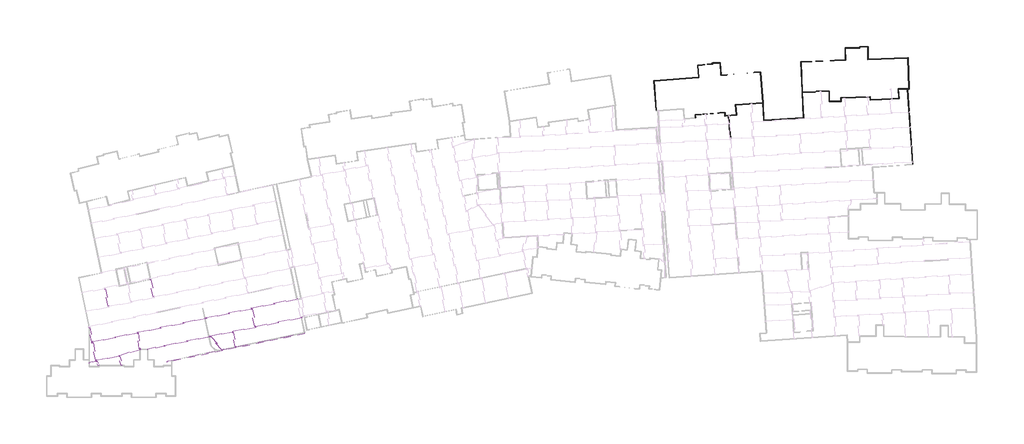
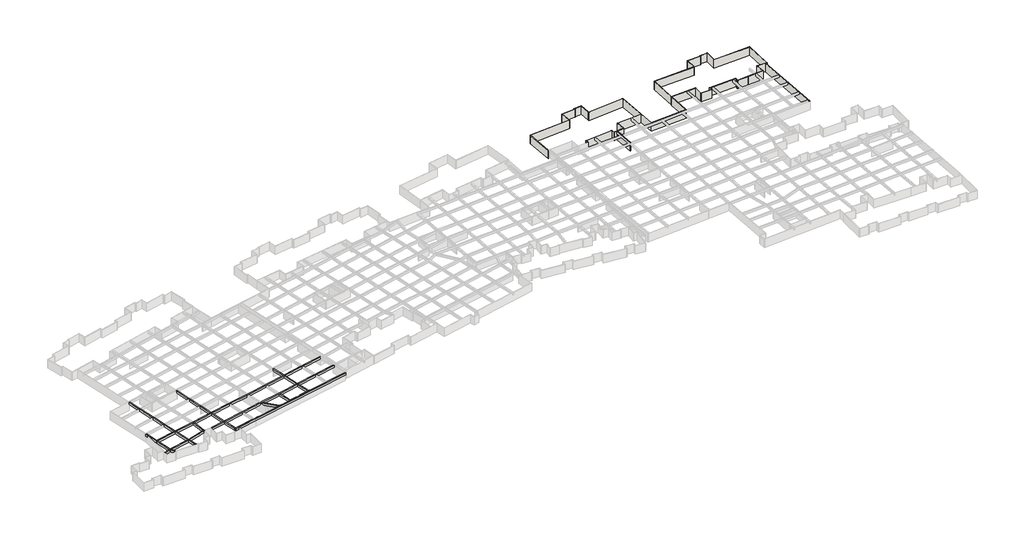
# One storey, part 7 of 14: 39 walls, 16 beams.
"""IFC4 building model written with IfcOpenShell, lengths in millimetres."""

from ifc_helpers import new_model, si_unit, frame, origin, origin_with_axes, place, context, project, spatial, polyline, outline, extrude, faceted_brep, element, save

model = new_model("IFC4")

# Units and contexts
model_context = context("Model", 3, world=origin())
ifc_project = project(units=[si_unit("LENGTHUNIT", "METRE", prefix="MILLI")], contexts=[model_context])

# Site, building, storey
site = spatial("IfcSite", under=ifc_project)
building = spatial("IfcBuilding", under=site)
storey = spatial("IfcBuildingStorey", under=building, Name="户型图", Elevation=0.0)

# Beams
placement = place(None, origin())
element("IfcBeam", 1, ObjectType="混凝土 - 矩形梁 : KL_beam", at=placement, inside=storey, context=model_context, shape_type="Brep", body=[
    faceted_brep([(-263201.3012877, -185738.5958614, 3300.0), (-263118.1366114, -186129.8549017, 3300.0), (-263118.1366114, -186129.8549017, 2500.0), (-263201.3012877, -185738.5958614, 2500.0), (-270867.2111578, -187368.0353054, 3300.0), (-271258.4701981, -187451.1999817, 3300.0), (-278694.4077882, -189031.7573087, 3300.0), (-279085.6668285, -189114.921985, 3300.0), (-286512.5798142, -190693.5610731, 3300.0), (-286903.8388545, -190776.7257494, 3300.0), (-294373.2864186, -192364.4058412, 3300.0), (-294764.5454589, -192447.5705175, 3300.0), (-302149.0676913, -194017.1991728, 3300.0), (-302540.3269101, -194100.3638871, 3300.0), (-310014.318982, -195689.0099438, 3300.0), (-310405.5780223, -195772.1746202, 3300.0), (-317795.331615, -197342.9152354, 3300.0), (-318186.5906553, -197426.0799118, 3300.0), (-325566.4629617, -198994.7201948, 3300.0), (-325957.722002, -199077.8848711, 3300.0), (-333450.1072491, -200670.4405179, 3300.0), (-333841.3662894, -200753.6051942, 3300.0), (-333758.2016131, -201144.8642345, 3300.0), (-333366.9425728, -201061.6995582, 3300.0), (-325874.5573256, -199469.1439114, 3300.0), (-325483.2982853, -199385.979235, 3300.0), (-318121.2886173, -197821.135773, 3300.0), (-317728.535031, -197737.6534211, 3300.0), (-310322.4133459, -196163.4336605, 3300.0), (-309931.1543056, -196080.2689841, 3300.0), (-302456.7885265, -194491.5434934, 3300.0), (-302065.5293077, -194408.3787792, 3300.0), (-294681.3807826, -192838.8295578, 3300.0), (-294290.1217423, -192755.6648815, 3300.0), (-286820.6741782, -191167.9847897, 3300.0), (-286429.4151379, -191084.8201134, 3300.0), (-279002.5021521, -189506.1810253, 3300.0), (-278611.2431118, -189423.016349, 3300.0), (-271175.3055217, -187842.459022, 3300.0), (-270784.0464815, -187759.2943457, 3300.0), (-333758.2016131, -201144.8642345, 2500.0), (-333366.9425728, -201061.6995582, 2500.0), (-325874.5573256, -199469.1439114, 2500.0), (-325483.2982853, -199385.979235, 2500.0), (-318121.2886173, -197821.135773, 2500.0), (-317728.535031, -197737.6534211, 2500.0), (-310322.4133459, -196163.4336605, 2500.0), (-309931.1543056, -196080.2689841, 2500.0), (-302456.7885265, -194491.5434934, 2500.0), (-302065.5293077, -194408.3787792, 2500.0), (-294681.3807826, -192838.8295578, 2500.0), (-294290.1217423, -192755.6648815, 2500.0), (-286820.6741782, -191167.9847897, 2500.0), (-286429.4151379, -191084.8201134, 2500.0), (-279002.5021521, -189506.1810253, 2500.0), (-278611.2431118, -189423.016349, 2500.0), (-271175.3055217, -187842.459022, 2500.0), (-270784.0464815, -187759.2943457, 2500.0), (-333841.3662894, -200753.6051942, 2500.0), (-333450.1072491, -200670.4405179, 2500.0), (-325957.722002, -199077.8848711, 2500.0), (-325566.4629617, -198994.7201948, 2500.0), (-318186.5906553, -197426.0799118, 2500.0), (-317795.331615, -197342.9152354, 2500.0), (-310405.5780223, -195772.1746202, 2500.0), (-310014.318982, -195689.0099438, 2500.0), (-302540.3269101, -194100.3638871, 2500.0), (-302149.0676913, -194017.1991728, 2500.0), (-294764.5454589, -192447.5705175, 2500.0), (-294373.2864186, -192364.4058412, 2500.0), (-286903.8388545, -190776.7257494, 2500.0), (-286512.5798142, -190693.5610731, 2500.0), (-279085.6668285, -189114.921985, 2500.0), (-278694.4077882, -189031.7573087, 2500.0), (-271258.4701981, -187451.1999817, 2500.0), (-270867.2111578, -187368.0353054, 2500.0)], [[[0, 1, 2, 3]], [[1, 0, 4, 5, 6, 7, 8, 9, 10, 11, 12, 13, 14, 15, 16, 17, 18, 19, 20, 21, 22, 23, 24, 25, 26, 27, 28, 29, 30, 31, 32, 33, 34, 35, 36, 37, 38, 39]], [[2, 1, 39, 38, 37, 36, 35, 34, 33, 32, 31, 30, 29, 28, 27, 26, 25, 24, 23, 22, 40, 41, 42, 43, 44, 45, 46, 47, 48, 49, 50, 51, 52, 53, 54, 55, 56, 57]], [[3, 2, 57, 56, 55, 54, 53, 52, 51, 50, 49, 48, 47, 46, 45, 44, 43, 42, 41, 40, 58, 59, 60, 61, 62, 63, 64, 65, 66, 67, 68, 69, 70, 71, 72, 73, 74, 75]], [[0, 3, 75, 74, 73, 72, 71, 70, 69, 68, 67, 66, 65, 64, 63, 62, 61, 60, 59, 58, 21, 20, 19, 18, 17, 16, 15, 14, 13, 12, 11, 10, 9, 8, 7, 6, 5, 4]], [[22, 21, 58, 40]]]),
])
element("IfcBeam", 2, ObjectType="混凝土 - 矩形梁 : KL_beam", at=placement, inside=storey, context=model_context, shape_type="Brep", body=[
    faceted_brep([(-324374.5463738, -205804.6094179, 3300.0), (-324476.8521438, -205417.4189427, 3300.0), (-324604.4476356, -205444.5402017, 3300.0), (-332096.8328827, -207037.0958485, 3300.0), (-332488.091923, -207120.2605249, 3300.0), (-332483.9504903, -207139.7444339, 3300.0), (-332404.9272467, -207511.5195652, 3300.0), (-332199.0452178, -207467.757989, 3300.0), (-331946.3573579, -207414.0475263, 3300.0), (-324510.9984157, -205833.6131948, 3300.0), (-324374.5463738, -205804.6094179, 2500.0), (-332404.9272467, -207511.5195652, 2500.0), (-332199.0452178, -207467.757989, 2500.0), (-331946.3573579, -207414.0475263, 2500.0), (-324510.9984157, -205833.6131948, 2500.0), (-324476.8521438, -205417.4189427, 2500.0), (-332483.9504903, -207139.7444339, 2500.0), (-332488.091923, -207120.2605249, 2500.0), (-332096.8328827, -207037.0958485, 2500.0), (-324604.4476356, -205444.5402017, 2500.0)], [[[0, 1, 2, 3, 4, 5, 6, 7, 8, 9]], [[10, 0, 9, 8, 7, 6, 11, 12, 13, 14]], [[15, 10, 14, 13, 12, 11, 16, 17, 18, 19]], [[1, 15, 19, 18, 17, 4, 3, 2]], [[1, 0, 10, 15]], [[6, 5, 4, 17, 16, 11]]]),
])
element("IfcBeam", 3, ObjectType="混凝土 - 矩形梁 : KL_beam", at=placement, inside=storey, context=model_context, shape_type="Brep", body=[
    faceted_brep([(-324476.8521438, -205417.4189427, 3300.0), (-324374.5463738, -205804.6094179, 3300.0), (-324125.8041879, -205725.6963015, 3300.0), (-317024.3512452, -203472.7701219, 3300.0), (-317073.94554, -203068.8570036, 3300.0), (-317461.8397372, -203191.9159042, 3300.0), (-324218.6852395, -205335.5158473, 3300.0), (-324374.5463738, -205804.6094179, 2500.0), (-324125.8041879, -205725.6963015, 2500.0), (-317024.3512452, -203472.7701219, 2500.0), (-324476.8521438, -205417.4189427, 2500.0), (-324218.6852395, -205335.5158473, 2500.0), (-317461.8397372, -203191.9159042, 2500.0), (-317073.94554, -203068.8570036, 2500.0)], [[[0, 1, 2, 3, 4, 5, 6]], [[1, 7, 8, 9, 3, 2]], [[7, 10, 11, 12, 13, 9, 8]], [[10, 0, 6, 5, 4, 13, 12, 11]], [[0, 10, 7, 1]], [[4, 3, 9, 13]]]),
])
element("IfcBeam", 4, ObjectType="混凝土 - 矩形梁 : KL_beam", at=placement, inside=storey, context=model_context, shape_type="Brep", body=[
    faceted_brep([(-314583.4302282, -203136.4522332, 3300.0), (-314583.4302282, -203136.4522332, 2500.0), (-314502.1811132, -203528.1135426, 2500.0), (-314502.1811132, -203528.1135426, 3300.0), (-261465.8556991, -192525.8664512, 3300.0), (-261547.1048141, -192134.2051418, 3300.0), (-261938.9355731, -192215.4894087, 3300.0), (-269503.3072813, -193784.6985493, 3300.0), (-269894.9732799, -193865.948637, 3300.0), (-277338.6451756, -195410.118917, 3300.0), (-277730.3111743, -195491.3690048, 3300.0), (-285164.9490789, -197033.6652069, 3300.0), (-285556.6150776, -197114.9152947, 3300.0), (-293033.8318018, -198666.0443617, 3300.0), (-293425.4978005, -198747.2944494, 3300.0), (-300811.7120035, -200279.5452813, 3300.0), (-301203.3800115, -200360.7957858, 3300.0), (-308691.1329963, -201914.1105725, 3300.0), (-309082.7989949, -201995.3606603, 3300.0), (-308999.6333229, -202386.624385, 3300.0), (-308607.9673243, -202305.3742972, 3300.0), (-301119.8402372, -200751.981904, 3300.0), (-300728.1722293, -200670.7313994, 3300.0), (-293255.3826053, -199120.5207228, 3300.0), (-292792.1219887, -199024.4185187, 3300.0), (-285474.4053395, -197506.3773254, 3300.0), (-285082.74403, -197425.1282104, 3300.0), (-277647.1455022, -195882.6327295, 3300.0), (-277255.4795036, -195801.3826417, 3300.0), (-269811.8076079, -194257.2123617, 3300.0), (-269420.1416092, -194175.962274, 3300.0), (-261465.8556991, -192525.8664512, 2500.0), (-308999.6333229, -202386.624385, 2500.0), (-308607.9673243, -202305.3742972, 2500.0), (-301119.8402372, -200751.981904, 2500.0), (-300728.1722293, -200670.7313994, 2500.0), (-293255.3826053, -199120.5207228, 2500.0), (-292792.1219887, -199024.4185187, 2500.0), (-285474.4053395, -197506.3773254, 2500.0), (-285082.74403, -197425.1282104, 2500.0), (-277647.1455022, -195882.6327295, 2500.0), (-277255.4795036, -195801.3826417, 2500.0), (-269811.8076079, -194257.2123617, 2500.0), (-269420.1416092, -194175.962274, 2500.0), (-261547.1048141, -192134.2051418, 2500.0), (-309082.7989949, -201995.3606603, 2500.0), (-308691.1329963, -201914.1105725, 2500.0), (-301203.3800115, -200360.7957858, 2500.0), (-300811.7120035, -200279.5452813, 2500.0), (-293425.4978005, -198747.2944494, 2500.0), (-293033.8318018, -198666.0443617, 2500.0), (-285556.6150776, -197114.9152947, 2500.0), (-285164.9490789, -197033.6652069, 2500.0), (-277730.3111743, -195491.3690048, 2500.0), (-277338.6451756, -195410.118917, 2500.0), (-269894.9732799, -193865.948637, 2500.0), (-269503.3072813, -193784.6985493, 2500.0), (-261938.9355731, -192215.4894087, 2500.0)], [[[0, 1, 2, 3]], [[4, 5, 6, 7, 8, 9, 10, 11, 12, 13, 14, 15, 16, 17, 18, 0, 3, 19, 20, 21, 22, 23, 24, 25, 26, 27, 28, 29, 30]], [[31, 4, 30, 29, 28, 27, 26, 25, 24, 23, 22, 21, 20, 19, 3, 2, 32, 33, 34, 35, 36, 37, 38, 39, 40, 41, 42, 43]], [[44, 31, 43, 42, 41, 40, 39, 38, 37, 36, 35, 34, 33, 32, 2, 1, 45, 46, 47, 48, 49, 50, 51, 52, 53, 54, 55, 56, 57]], [[5, 44, 57, 56, 55, 54, 53, 52, 51, 50, 49, 48, 47, 46, 45, 1, 0, 18, 17, 16, 15, 14, 13, 12, 11, 10, 9, 8, 7, 6]], [[5, 4, 31, 44]]]),
])
element("IfcBeam", 5, ObjectType="混凝土 - 矩形梁 : KL_beam", at=placement, inside=storey, context=model_context, shape_type="Brep", body=[
    faceted_brep([(-260736.4967976, -197615.6911599, 3300.0), (-260655.2476826, -198007.3524693, 3300.0), (-260655.2476826, -198007.3524693, 2500.0), (-260736.4967976, -197615.6911599, 2500.0), (-268353.1534946, -199195.7466848, 3300.0), (-268744.8194932, -199276.9967726, 3300.0), (-276188.4913889, -200821.1670525, 3300.0), (-276580.1573876, -200902.4171403, 3300.0), (-284040.3447093, -202450.0135022, 3300.0), (-284432.0060187, -202531.2626172, 3300.0), (-288575.5312118, -203390.826089, 3300.0), (-289038.7918284, -203486.9282932, 3300.0), (-299656.3845067, -205689.5201441, 3300.0), (-300048.0525146, -205770.7706487, 3300.0), (-307540.9792096, -207325.158708, 3300.0), (-307932.6452082, -207406.4087958, 3300.0), (-307849.4795362, -207797.6725205, 3300.0), (-307849.4795362, -207797.6725205, 2500.0), (-307932.6452082, -207406.4087958, 2500.0), (-307540.9792096, -207325.158708, 2500.0), (-300048.0525146, -205770.7706487, 2500.0), (-299656.3845067, -205689.5201441, 2500.0), (-289038.7918284, -203486.9282932, 2500.0), (-288575.5312118, -203390.826089, 2500.0), (-284432.0060187, -202531.2626172, 2500.0), (-284040.3447093, -202450.0135022, 2500.0), (-276580.1573876, -200902.4171403, 2500.0), (-276188.4913889, -200821.1670525, 2500.0), (-268744.8194932, -199276.9967726, 2500.0), (-268353.1534946, -199195.7466848, 2500.0)], [[[0, 1, 2, 3]], [[1, 0, 4, 5, 6, 7, 8, 9, 10, 11, 12, 13, 14, 15, 16]], [[2, 1, 16, 17]], [[3, 2, 17, 18, 19, 20, 21, 22, 23, 24, 25, 26, 27, 28, 29]], [[0, 3, 29, 28, 27, 26, 25, 24, 23, 22, 21, 20, 19, 18, 15, 14, 13, 12, 11, 10, 9, 8, 7, 6, 5, 4]], [[16, 15, 18, 17]]]),
])
element("IfcBeam", 6, ObjectType="混凝土 - 矩形梁 : KL_beam", at=placement, inside=storey, context=model_context, shape_type="SweptSolid", body=[
    extrude(outline(polyline([(-293255.3826053, -199120.5207228), (-292792.1219887, -199024.4185187), (-288575.5312118, -203390.826089), (-289038.7918284, -203486.9282932), (-293255.3826053, -199120.5207228)])), frame((0.0, 0.0, 2500.0), z_axis=(0.0, 0.0, 1.0), x_axis=(1.0, 0.0, 0.0)), (0.0, 0.0, 1.0), 800.0),
])
element("IfcBeam", 7, ObjectType="混凝土 - 矩形梁 : KL_beam", at=placement, inside=storey, context=model_context, shape_type="SweptSolid", body=[
    extrude(outline(polyline([(-285474.4053395, -197506.3773254), (-285082.74403, -197425.1282104), (-284040.3447093, -202450.0135022), (-284432.0060187, -202531.2626172), (-285474.4053395, -197506.3773254)])), frame((0.0, 0.0, 2500.0), z_axis=(0.0, 0.0, 1.0), x_axis=(1.0, 0.0, 0.0)), (0.0, 0.0, 1.0), 800.0),
])
element("IfcBeam", 8, ObjectType="混凝土 - 矩形梁 : KL_beam", at=placement, inside=storey, context=model_context, shape_type="SweptSolid", body=[
    extrude(outline(polyline([(-280137.7839447, -184165.1001211), (-279746.5249044, -184081.9354447), (-278694.4077882, -189031.7573087), (-279085.6668285, -189114.921985), (-280137.7839447, -184165.1001211)])), frame((0.0, 0.0, 2500.0), z_axis=(0.0, 0.0, 1.0), x_axis=(1.0, 0.0, 0.0)), (0.0, 0.0, 1.0), 800.0),
    extrude(outline(polyline([(-276188.4913889, -200821.1670525), (-276580.1573876, -200902.4171403), (-277647.1455022, -195882.6327295), (-277255.4795036, -195801.3826417), (-276188.4913889, -200821.1670525)])), frame((0.0, 0.0, 2500.0), z_axis=(0.0, 0.0, 1.0), x_axis=(1.0, 0.0, 0.0)), (0.0, 0.0, 1.0), 800.0),
    extrude(outline(polyline([(-279002.5021521, -189506.1810253), (-278611.2431118, -189423.016349), (-277338.6451756, -195410.118917), (-277730.3111743, -195491.3690048), (-279002.5021521, -189506.1810253)])), frame((0.0, 0.0, 2500.0), z_axis=(0.0, 0.0, 1.0), x_axis=(1.0, 0.0, 0.0)), (0.0, 0.0, 1.0), 800.0),
])
element("IfcBeam", 9, ObjectType="混凝土 - 矩形梁 : KL_beam", at=placement, inside=storey, context=model_context, shape_type="SweptSolid", body=[
    extrude(outline(polyline([(-313895.401585, -179353.84561), (-313504.1425447, -179270.6809336), (-312251.5327359, -185163.7467557), (-312642.7917762, -185246.9114321), (-313895.401585, -179353.84561)])), frame((0.0, 0.0, 2500.0), z_axis=(0.0, 0.0, 1.0), x_axis=(1.0, 0.0, 0.0)), (0.0, 0.0, 1.0), 800.0),
    extrude(outline(polyline([(-307540.9792096, -207325.158708), (-307932.6452082, -207406.4087958), (-308999.6333229, -202386.624385), (-308607.9673243, -202305.3742972), (-307540.9792096, -207325.158708)])), frame((0.0, 0.0, 2500.0), z_axis=(0.0, 0.0, 1.0), x_axis=(1.0, 0.0, 0.0)), (0.0, 0.0, 1.0), 800.0),
    extrude(outline(polyline([(-312559.6270999, -185638.1704723), (-312168.3680596, -185555.005796), (-311149.6007746, -190347.9290396), (-311540.8598149, -190431.0937159), (-312559.6270999, -185638.1704723)])), frame((0.0, 0.0, 2500.0), z_axis=(0.0, 0.0, 1.0), x_axis=(1.0, 0.0, 0.0)), (0.0, 0.0, 1.0), 800.0),
    extrude(outline(polyline([(-311457.6951385, -190822.3527562), (-311066.4360982, -190739.1880799), (-310014.318982, -195689.0099438), (-310405.5780223, -195772.1746202), (-311457.6951385, -190822.3527562)])), frame((0.0, 0.0, 2500.0), z_axis=(0.0, 0.0, 1.0), x_axis=(1.0, 0.0, 0.0)), (0.0, 0.0, 1.0), 800.0),
    extrude(outline(polyline([(-310322.4133459, -196163.4336605), (-309931.1543056, -196080.2689841), (-308691.1329963, -201914.1105725), (-309082.7989949, -201995.3606603), (-310322.4133459, -196163.4336605)])), frame((0.0, 0.0, 2500.0), z_axis=(0.0, 0.0, 1.0), x_axis=(1.0, 0.0, 0.0)), (0.0, 0.0, 1.0), 800.0),
])
element("IfcBeam", 10, ObjectType="混凝土 - 矩形梁 : KL_beam", at=placement, inside=storey, context=model_context, shape_type="SweptSolid", body=[
    extrude(outline(polyline([(-317073.94554, -203068.8570036), (-317461.8397372, -203191.9159042), (-318121.2886173, -197821.135773), (-317728.535031, -197737.6534211), (-317073.94554, -203068.8570036)])), frame((0.0, 0.0, 2500.0), z_axis=(0.0, 0.0, 1.0), x_axis=(1.0, 0.0, 0.0)), (0.0, 0.0, 1.0), 800.0),
])
element("IfcBeam", 11, ObjectType="混凝土 - 矩形梁 : KL_beam", at=placement, inside=storey, context=model_context, shape_type="SweptSolid", body=[
    extrude(outline(polyline([(-324218.6852395, -205335.5158473), (-324476.8521438, -205417.4189427), (-324604.4476356, -205444.5402017), (-325874.5573256, -199469.1439114), (-325483.2982853, -199385.979235), (-324218.6852395, -205335.5158473)])), frame((0.0, 0.0, 2500.0), z_axis=(0.0, 0.0, 1.0), x_axis=(1.0, 0.0, 0.0)), (0.0, 0.0, 1.0), 800.0),
    extrude(outline(polyline([(-330589.6253093, -177286.4931074), (-330198.366269, -177203.3284311), (-329172.7701325, -182028.3788949), (-329564.0291728, -182111.5435712), (-330589.6253093, -177286.4931074)])), frame((0.0, 0.0, 2500.0), z_axis=(0.0, 0.0, 1.0), x_axis=(1.0, 0.0, 0.0)), (0.0, 0.0, 1.0), 800.0),
    extrude(outline(polyline([(-329480.8644965, -182502.8026115), (-329089.6054562, -182419.6379352), (-327803.6767156, -188469.4570066), (-328194.9357559, -188552.621683), (-329480.8644965, -182502.8026115)])), frame((0.0, 0.0, 2500.0), z_axis=(0.0, 0.0, 1.0), x_axis=(1.0, 0.0, 0.0)), (0.0, 0.0, 1.0), 800.0),
    extrude(outline(polyline([(-328111.7710796, -188943.8807233), (-327720.5120393, -188860.7160469), (-326701.7447543, -193653.6392905), (-327093.0037946, -193736.8039669), (-328111.7710796, -188943.8807233)])), frame((0.0, 0.0, 2500.0), z_axis=(0.0, 0.0, 1.0), x_axis=(1.0, 0.0, 0.0)), (0.0, 0.0, 1.0), 800.0),
    extrude(outline(polyline([(-327009.8391182, -194128.0630072), (-326618.580078, -194044.8983308), (-325566.4629617, -198994.7201948), (-325957.722002, -199077.8848711), (-327009.8391182, -194128.0630072)])), frame((0.0, 0.0, 2500.0), z_axis=(0.0, 0.0, 1.0), x_axis=(1.0, 0.0, 0.0)), (0.0, 0.0, 1.0), 800.0),
])
element("IfcBeam", 12, ObjectType="混凝土 - 矩形梁 : KL_beam", at=placement, inside=storey, context=model_context, shape_type="SweptSolid", body=[
    extrude(outline(polyline([(-333758.2016131, -201144.8642345), (-333366.9425728, -201061.6995582), (-332096.8328827, -207037.0958485), (-332488.091923, -207120.2605249), (-333758.2016131, -201144.8642345)])), frame((0.0, 0.0, 2500.0), z_axis=(0.0, 0.0, 1.0), x_axis=(1.0, 0.0, 0.0)), (0.0, 0.0, 1.0), 800.0),
])
element("IfcBeam", 13, ObjectType="混凝土 - 矩形梁 : KL_beam", at=placement, inside=storey, context=model_context, shape_type="SweptSolid", body=[
    extrude(outline(polyline([(-334893.4834057, -195803.7833303), (-334502.2243654, -195720.618654), (-333450.1072491, -200670.4405179), (-333841.3662894, -200753.6051942), (-334893.4834057, -195803.7833303)])), frame((0.0, 0.0, 2500.0), z_axis=(0.0, 0.0, 1.0), x_axis=(1.0, 0.0, 0.0)), (0.0, 0.0, 1.0), 800.0),
])
element("IfcBeam", 14, ObjectType="混凝土 - 矩形梁 : KL_beam", at=placement, inside=storey, context=model_context, shape_type="Brep", body=[
    faceted_brep([(-334581.1379592, -208241.7468389, 3300.0), (-334704.7447569, -207861.3242324, 3300.0), (-334704.7447569, -207861.3242324, 2500.0), (-334581.1379592, -208241.7468389, 2500.0), (-332346.7102012, -207515.7372506, 3300.0), (-332199.0452178, -207467.757989, 3300.0), (-332404.9272467, -207511.5195652, 3300.0), (-332483.9504903, -207139.7444339, 3300.0), (-332483.9504903, -207139.7444339, 2500.0), (-332404.9272467, -207511.5195652, 2500.0), (-332199.0452178, -207467.757989, 2500.0), (-332346.7102012, -207515.7372506, 2500.0)], [[[0, 1, 2, 3]], [[1, 0, 4, 5, 6, 7]], [[2, 1, 7, 8]], [[3, 2, 8, 9, 10, 11]], [[0, 3, 11, 10, 5, 4]], [[9, 6, 5, 10]], [[6, 9, 8, 7]]]),
])
element("IfcBeam", 15, ObjectType="混凝土 - 矩形梁 : KL_beam", at=placement, inside=storey, context=model_context, shape_type="Brep", body=[
    faceted_brep([(-331167.7348677, -208836.1730889, 3300.0), (-331518.5900609, -209028.2684646, 3300.0), (-331518.5900609, -209028.2684646, 2500.0), (-331167.7348677, -208836.1730889, 2500.0), (-331946.3573579, -207414.0475263, 3300.0), (-332013.6682064, -207428.3548888, 3300.0), (-332199.0452178, -207467.757989, 3300.0), (-332346.7102012, -207515.7372506, 3300.0), (-332346.7102012, -207515.7372506, 2500.0), (-332199.0452178, -207467.757989, 2500.0), (-332013.6682064, -207428.3548888, 2500.0), (-331946.3573579, -207414.0475263, 2500.0)], [[[0, 1, 2, 3]], [[1, 0, 4, 5, 6, 7]], [[2, 1, 7, 8]], [[3, 2, 8, 9, 10, 11]], [[0, 3, 11, 4]], [[4, 11, 10, 9, 6, 5]], [[7, 6, 9, 8]]]),
])
element("IfcBeam", 16, ObjectType="混凝土 - 矩形梁 : KL_beam", at=placement, inside=storey, context=model_context, shape_type="Brep", body=[
    faceted_brep([(-323307.349972, -208780.209019, 3300.0), (-323693.7203025, -208883.736637, 3300.0), (-323693.7203025, -208883.736637, 2500.0), (-323307.349972, -208780.209019, 2500.0), (-324125.8041879, -205725.6963015, 3300.0), (-324135.1215252, -205728.652214, 3300.0), (-324374.5463738, -205804.6094179, 3300.0), (-324510.9984157, -205833.6131948, 3300.0), (-324510.9984157, -205833.6131948, 2500.0), (-324374.5463738, -205804.6094179, 2500.0), (-324135.1215252, -205728.652214, 2500.0), (-324125.8041879, -205725.6963015, 2500.0)], [[[0, 1, 2, 3]], [[1, 0, 4, 5, 6, 7]], [[2, 1, 7, 8]], [[3, 2, 8, 9, 10, 11]], [[0, 3, 11, 4]], [[4, 11, 10, 9, 6, 5]], [[7, 6, 9, 8]]]),
])

# Walls
element("IfcWall", 17, ObjectType="所有墙体", at=placement, inside=storey, context=model_context, shape_type="Brep", body=[
    faceted_brep([(-89521.5287585, -114818.9842862, 0.0), (-89520.4912267, -114818.9480548, 0.0), (-89400.5460592, -114814.7594773, 0.0), (-80206.4694387, -114493.6952469, 0.0), (-80086.4694387, -114489.5047546, 0.0), (-80086.4694387, -114489.5047546, 3300.0), (-80206.4694387, -114493.6952469, 3300.0), (-89400.5460592, -114814.7594773, 3300.0), (-89520.4912267, -114818.9480548, 3300.0), (-89521.5287585, -114818.9842862, 3300.0), (-89525.7166981, -114699.057387, 0.0), (-89525.7166981, -114699.057387, 3300.0), (-89405.7897988, -114694.8694474, 3300.0), (-80086.4694387, -114369.4316093, 3300.0), (-80086.4694387, -114369.4316093, 0.0), (-89405.7897988, -114694.8694474, 0.0)], [[[0, 1, 2, 3, 4, 5, 6, 7, 8, 9]], [[10, 11, 12, 13, 14, 15]], [[4, 3, 2, 1, 0, 10, 15, 14]], [[9, 8, 7, 6, 5, 13, 12, 11]], [[5, 4, 14, 13]], [[0, 9, 11, 10]]]),
])
element("IfcWall", 18, ObjectType="所有墙体", at=placement, inside=storey, context=model_context, shape_type="Brep", body=[
    faceted_brep([(-80206.4694387, -114493.6952469, 0.0), (-80206.4694387, -117991.5634281, 0.0), (-80206.4694387, -117991.5634281, 3300.0), (-80206.4694387, -114493.6952469, 3300.0), (-80086.4694387, -114489.5047546, 0.0), (-80086.4694387, -114489.5047546, 3300.0), (-80086.4694387, -117871.5634281, 3300.0), (-80086.4694387, -117991.5634281, 3300.0), (-80086.4694387, -117991.5634281, 0.0), (-80086.4694387, -117871.5634281, 0.0)], [[[0, 1, 2, 3]], [[4, 5, 6, 7, 8, 9]], [[1, 0, 4, 9, 8]], [[3, 2, 7, 6, 5]], [[0, 3, 5, 4]], [[2, 1, 8, 7]]]),
])
element("IfcWall", 19, ObjectType="所有墙体", at=placement, inside=storey, context=model_context, shape_type="Brep", body=[
    faceted_brep([(-80086.4694387, -117991.5634281, 0.0), (-76086.4694387, -117991.5634281, 0.0), (-76086.4694387, -117991.5634281, 3300.0), (-80086.4694387, -117991.5634281, 3300.0), (-80086.4694387, -117871.5634281, 0.0), (-80086.4694387, -117871.5634281, 3300.0), (-76206.4694387, -117871.5634281, 3300.0), (-76086.4694387, -117871.5634281, 3300.0), (-76086.4694387, -117871.5634281, 0.0), (-76206.4694387, -117871.5634281, 0.0)], [[[0, 1, 2, 3]], [[4, 5, 6, 7, 8, 9]], [[1, 0, 4, 9, 8]], [[3, 2, 7, 6, 5]], [[0, 3, 5, 4]], [[2, 1, 8, 7]]]),
])
element("IfcWall", 20, ObjectType="所有墙体", at=placement, inside=storey, context=model_context, shape_type="Brep", body=[
    faceted_brep([(-76086.4694387, -117871.5634281, 0.0), (-76086.4694387, -116784.9907166, 0.0), (-76086.4694387, -116664.9175713, 0.0), (-76086.4694387, -116664.9175713, 3300.0), (-76086.4694387, -116784.9907166, 3300.0), (-76086.4694387, -117871.5634281, 3300.0), (-76206.4694387, -117871.5634281, 0.0), (-76206.4694387, -117871.5634281, 3300.0), (-76206.4694387, -116669.1080636, 3300.0), (-76206.4694387, -116669.1080636, 0.0)], [[[0, 1, 2, 3, 4, 5]], [[6, 7, 8, 9]], [[2, 1, 0, 6, 9]], [[5, 4, 3, 8, 7]], [[0, 5, 7, 6]], [[3, 2, 9, 8]]]),
])
element("IfcWall", 21, ObjectType="所有墙体", at=placement, inside=storey, context=model_context, shape_type="Brep", body=[
    faceted_brep([(-76086.4694387, -116784.9907166, 0.0), (-66112.6220858, -116436.6962923, 0.0), (-65992.6220858, -116432.5057999, 0.0), (-65992.6220858, -116432.5057999, 3300.0), (-66112.6220858, -116436.6962923, 3300.0), (-76086.4694387, -116784.9907166, 3300.0), (-76086.4694387, -116664.9175713, 0.0), (-76086.4694387, -116664.9175713, 3300.0), (-65992.6220858, -116312.4326546, 3300.0), (-65992.6220858, -116312.4326546, 0.0)], [[[0, 1, 2, 3, 4, 5]], [[6, 7, 8, 9]], [[2, 1, 0, 6, 9]], [[5, 4, 3, 8, 7]], [[0, 5, 7, 6]], [[3, 2, 9, 8]]]),
])
element("IfcWall", 22, ObjectType="所有墙体", at=placement, inside=storey, context=model_context, shape_type="Brep", body=[
    faceted_brep([(-66112.6220858, -116436.6962923, 0.0), (-66112.6220858, -117536.6962923, 0.0), (-66112.6220858, -117536.6962923, 3300.0), (-66112.6220858, -116436.6962923, 3300.0), (-65992.6220858, -116432.5057999, 0.0), (-65992.6220858, -116432.5057999, 3300.0), (-65992.6220858, -117412.4326546, 3300.0), (-65992.6220858, -117532.5057999, 3300.0), (-65992.6220858, -117532.5057999, 0.0), (-65992.6220858, -117412.4326546, 0.0)], [[[0, 1, 2, 3]], [[4, 5, 6, 7, 8, 9]], [[1, 0, 4, 9, 8]], [[3, 2, 7, 6, 5]], [[0, 3, 5, 4]], [[2, 1, 8, 7]]]),
])
element("IfcWall", 23, ObjectType="所有墙体", at=placement, inside=storey, context=model_context, shape_type="SweptSolid", body=[
    extrude(outline(polyline([(-62032.4536983, -117394.2136725), (-65992.6220858, -117532.5057999), (-65992.6220858, -117412.4326546), (-62037.6882241, -117274.3233209), (-62032.4536983, -117394.2136725)])), origin_with_axes(), (0.0, 0.0, 1.0), 3300.0),
])
element("IfcWall", 24, ObjectType="所有墙体", at=placement, inside=storey, context=model_context, shape_type="Brep", body=[
    faceted_brep([(-62032.4536983, -117394.2136725, 0.0), (-56077.9698795, -117082.1523988, 0.0), (-56077.9698795, -117082.1523988, 3300.0), (-62032.4536983, -117394.2136725, 3300.0), (-62037.6882241, -117274.3233209, 0.0), (-62037.6882241, -117274.3233209, 3300.0), (-56208.3435329, -116968.8203109, 3300.0), (-56088.4349436, -116962.536168, 3300.0), (-56088.4349436, -116962.536168, 0.0), (-56208.3435329, -116968.8203109, 0.0)], [[[0, 1, 2, 3]], [[4, 5, 6, 7, 8, 9]], [[1, 0, 4, 9, 8]], [[3, 2, 7, 6, 5]], [[0, 3, 5, 4]], [[2, 1, 8, 7]]]),
])
element("IfcWall", 25, ObjectType="所有墙体", at=placement, inside=storey, context=model_context, shape_type="Brep", body=[
    faceted_brep([(-56088.4349436, -116962.536168, 0.0), (-56374.0077214, -113698.4243813, 0.0), (-56384.5063611, -113578.4243813, 0.0), (-56384.5063611, -113578.4243813, 3300.0), (-56374.0077214, -113698.4243813, 3300.0), (-56088.4349436, -116962.536168, 3300.0), (-56208.3435329, -116968.8203109, 0.0), (-56208.3435329, -116968.8203109, 3300.0), (-56504.9647416, -113578.4243813, 3300.0), (-56504.9647416, -113578.4243813, 0.0)], [[[0, 1, 2, 3, 4, 5]], [[6, 7, 8, 9]], [[2, 1, 0, 6, 9]], [[5, 4, 3, 8, 7]], [[0, 5, 7, 6]], [[3, 2, 9, 8]]]),
])
element("IfcWall", 26, ObjectType="所有墙体", at=placement, inside=storey, context=model_context, shape_type="Brep", body=[
    faceted_brep([(-56374.0077214, -113698.4243813, 0.0), (-53339.2709615, -113698.4243813, 0.0), (-53218.9779337, -113698.4243813, 0.0), (-52677.3544127, -113698.4243813, 0.0), (-52677.3544127, -113698.4243813, 3300.0), (-53218.9779337, -113698.4243813, 3300.0), (-53339.2709615, -113698.4243813, 3300.0), (-56374.0077214, -113698.4243813, 3300.0), (-56384.5063611, -113578.4243813, 0.0), (-56384.5063611, -113578.4243813, 3300.0), (-52801.6180503, -113578.4243813, 3300.0), (-52681.544905, -113578.4243813, 3300.0), (-52681.544905, -113578.4243813, 0.0), (-52801.6180503, -113578.4243813, 0.0)], [[[0, 1, 2, 3, 4, 5, 6, 7]], [[8, 9, 10, 11, 12, 13]], [[3, 2, 1, 0, 8, 13, 12]], [[7, 6, 5, 4, 11, 10, 9]], [[0, 7, 9, 8]], [[4, 3, 12, 11]]]),
])
element("IfcWall", 27, ObjectType="所有墙体", at=placement, inside=storey, context=model_context, shape_type="Brep", body=[
    faceted_brep([(-52681.544905, -113578.4243813, 0.0), (-53051.5514167, -102982.8241955, 0.0), (-53051.5514167, -102982.8241955, 3300.0), (-52681.544905, -113578.4243813, 3300.0), (-52801.6180503, -113578.4243813, 0.0), (-52801.6180503, -113578.4243813, 3300.0), (-53167.2903764, -103106.9390344, 3300.0), (-53171.478316, -102987.0121351, 3300.0), (-53171.478316, -102987.0121351, 0.0), (-53167.2903764, -103106.9390344, 0.0)], [[[0, 1, 2, 3]], [[4, 5, 6, 7, 8, 9]], [[1, 0, 4, 9, 8]], [[3, 2, 7, 6, 5]], [[0, 3, 5, 4]], [[2, 1, 8, 7]]]),
])
element("IfcWall", 28, ObjectType="所有墙体", at=placement, inside=storey, context=model_context, shape_type="Brep", body=[
    faceted_brep([(-53171.478316, -102987.0121351, 0.0), (-66829.4142289, -103463.9577669, 0.0), (-66949.4142289, -103468.1482592, 0.0), (-66949.4142289, -103468.1482592, 3300.0), (-66829.4142289, -103463.9577669, 3300.0), (-53171.478316, -102987.0121351, 3300.0), (-53167.2903764, -103106.9390344, 0.0), (-53167.2903764, -103106.9390344, 3300.0), (-66949.4142289, -103588.2214045, 3300.0), (-66949.4142289, -103588.2214045, 0.0)], [[[0, 1, 2, 3, 4, 5]], [[6, 7, 8, 9]], [[2, 1, 0, 6, 9]], [[5, 4, 3, 8, 7]], [[0, 5, 7, 6]], [[3, 2, 9, 8]]]),
])
element("IfcWall", 29, ObjectType="所有墙体", at=placement, inside=storey, context=model_context, shape_type="Brep", body=[
    faceted_brep([(-66829.4142289, -103463.9577669, 0.0), (-66829.4142289, -99066.0895857, 0.0), (-66829.4142289, -99066.0895857, 3300.0), (-66829.4142289, -103463.9577669, 3300.0), (-66949.4142289, -103468.1482592, 0.0), (-66949.4142289, -103468.1482592, 3300.0), (-66949.4142289, -99186.0895857, 3300.0), (-66949.4142289, -99066.0895857, 3300.0), (-66949.4142289, -99066.0895857, 0.0), (-66949.4142289, -99186.0895857, 0.0)], [[[0, 1, 2, 3]], [[4, 5, 6, 7, 8, 9]], [[1, 0, 4, 9, 8]], [[3, 2, 7, 6, 5]], [[0, 3, 5, 4]], [[2, 1, 8, 7]]]),
])
element("IfcWall", 30, ObjectType="所有墙体", at=placement, inside=storey, context=model_context, shape_type="Brep", body=[
    faceted_brep([(-66949.4142289, -99066.0895857, 0.0), (-69743.3156882, -99066.0895857, 0.0), (-69743.3156882, -99066.0895857, 3300.0), (-66949.4142289, -99066.0895857, 3300.0), (-66949.4142289, -99186.0895857, 0.0), (-66949.4142289, -99186.0895857, 3300.0), (-69623.3156882, -99186.0895857, 3300.0), (-69743.3156882, -99186.0895857, 3300.0), (-69743.3156882, -99186.0895857, 0.0), (-69623.3156882, -99186.0895857, 0.0)], [[[0, 1, 2, 3]], [[4, 5, 6, 7, 8, 9]], [[1, 0, 4, 9, 8]], [[3, 2, 7, 6, 5]], [[0, 3, 5, 4]], [[2, 1, 8, 7]]]),
])
element("IfcWall", 31, ObjectType="所有墙体", at=placement, inside=storey, context=model_context, shape_type="Brep", body=[
    faceted_brep([(-69743.3156882, -99186.0895857, 0.0), (-69743.3156882, -99548.8518078, 0.0), (-69743.3156882, -99668.8518078, 0.0), (-69743.3156882, -99668.8518078, 3300.0), (-69743.3156882, -99548.8518078, 3300.0), (-69743.3156882, -99186.0895857, 3300.0), (-69623.3156882, -99186.0895857, 0.0), (-69623.3156882, -99186.0895857, 3300.0), (-69623.3156882, -99668.8518078, 3300.0), (-69623.3156882, -99668.8518078, 0.0)], [[[0, 1, 2, 3, 4, 5]], [[6, 7, 8, 9]], [[2, 1, 0, 6, 9]], [[5, 4, 3, 8, 7]], [[0, 5, 7, 6]], [[3, 2, 9, 8]]]),
])
element("IfcWall", 32, ObjectType="所有墙体", at=placement, inside=storey, context=model_context, shape_type="Brep", body=[
    faceted_brep([(-69743.3156882, -99548.8518078, 0.0), (-74745.4475071, -99548.8518078, 0.0), (-74745.4475071, -99548.8518078, 3300.0), (-69743.3156882, -99548.8518078, 3300.0), (-69743.3156882, -99668.8518078, 0.0), (-69743.3156882, -99668.8518078, 3300.0), (-74621.1838694, -99668.8518078, 3300.0), (-74741.2570147, -99668.8518078, 3300.0), (-74741.2570147, -99668.8518078, 0.0), (-74621.1838694, -99668.8518078, 0.0)], [[[0, 1, 2, 3]], [[4, 5, 6, 7, 8, 9]], [[1, 0, 4, 9, 8]], [[3, 2, 7, 6, 5]], [[0, 3, 5, 4]], [[2, 1, 8, 7]]]),
])
element("IfcWall", 33, ObjectType="所有墙体", at=placement, inside=storey, context=model_context, shape_type="Brep", body=[
    faceted_brep([(-74741.2570147, -99668.8518078, 0.0), (-74599.2539845, -103735.28655, 0.0), (-74595.0660448, -103855.2134492, 0.0), (-74595.0660448, -103855.2134492, 3300.0), (-74599.2539845, -103735.28655, 3300.0), (-74741.2570147, -99668.8518078, 3300.0), (-74621.1838694, -99668.8518078, 0.0), (-74621.1838694, -99668.8518078, 3300.0), (-74475.1391456, -103851.0255096, 3300.0), (-74475.1391456, -103851.0255096, 0.0)], [[[0, 1, 2, 3, 4, 5]], [[6, 7, 8, 9]], [[2, 1, 0, 6, 9]], [[5, 4, 3, 8, 7]], [[0, 5, 7, 6]], [[3, 2, 9, 8]]]),
])
element("IfcWall", 34, ObjectType="所有墙体", at=placement, inside=storey, context=model_context, shape_type="Brep", body=[
    faceted_brep([(-74599.2539845, -103735.28655, 0.0), (-89889.9336378, -104269.2488495, 0.0), (-89889.9336378, -104269.2488495, 3300.0), (-74599.2539845, -103735.28655, 3300.0), (-74595.0660448, -103855.2134492, 0.0), (-74595.0660448, -103855.2134492, 3300.0), (-89765.818799, -104384.9878091, 3300.0), (-89885.7456982, -104389.1757487, 3300.0), (-89885.7456982, -104389.1757487, 0.0), (-89765.818799, -104384.9878091, 0.0)], [[[0, 1, 2, 3]], [[4, 5, 6, 7, 8, 9]], [[1, 0, 4, 9, 8]], [[3, 2, 7, 6, 5]], [[0, 3, 5, 4]], [[2, 1, 8, 7]]]),
])
element("IfcWall", 35, ObjectType="所有墙体", at=placement, inside=storey, context=model_context, shape_type="SweptSolid", body=[
    extrude(outline(polyline([(-89525.7166981, -114699.057387), (-89885.7456982, -104389.1757487), (-89765.818799, -104384.9878091), (-89405.7897988, -114694.8694474), (-89525.7166981, -114699.057387)])), origin_with_axes(), (0.0, 0.0, 1.0), 3300.0),
])
element("IfcWall", 36, ObjectType="所有墙体", at=placement, inside=storey, context=model_context, shape_type="Brep", body=[
    faceted_brep([(-89520.4912267, -114818.9480548, 0.0), (-89063.1839731, -123544.8902693, 0.0), (-89056.9032142, -123664.7342865, 0.0), (-89056.9032142, -123664.7342865, 3300.0), (-89063.1839731, -123544.8902693, 3300.0), (-89520.4912267, -114818.9480548, 3300.0), (-89400.5460592, -114814.7594773, 0.0), (-89400.5460592, -114814.7594773, 3300.0), (-88937.1423547, -123657.0289034, 3300.0), (-88937.1423547, -123657.0289034, 0.0)], [[[0, 1, 2, 3, 4, 5]], [[6, 7, 8, 9]], [[2, 1, 0, 6, 9]], [[5, 4, 3, 8, 7]], [[0, 5, 7, 6]], [[3, 2, 9, 8]]]),
])
element("IfcWall", 37, ObjectType="所有墙体", at=placement, inside=storey, context=model_context, shape_type="Brep", body=[
    faceted_brep([(-89063.1839731, -123544.8902693, 0.0), (-102615.1545701, -124416.8205942, 0.0), (-102734.9154296, -124424.5259773, 0.0), (-102734.9154296, -124424.5259773, 3300.0), (-102615.1545701, -124416.8205942, 3300.0), (-89063.1839731, -123544.8902693, 3300.0), (-89056.9032142, -123664.7342865, 0.0), (-89056.9032142, -123664.7342865, 3300.0), (-102728.6346708, -124544.3699945, 3300.0), (-102728.6346708, -124544.3699945, 0.0)], [[[0, 1, 2, 3, 4, 5]], [[6, 7, 8, 9]], [[2, 1, 0, 6, 9]], [[5, 4, 3, 8, 7]], [[0, 5, 7, 6]], [[3, 2, 9, 8]]]),
])
element("IfcWall", 38, ObjectType="所有墙体", at=placement, inside=storey, context=model_context, shape_type="Brep", body=[
    faceted_brep([(-102615.1545701, -124416.8205942, 0.0), (-102926.028435, -118484.993887, 0.0), (-102926.028435, -118484.993887, 3300.0), (-102615.1545701, -124416.8205942, 3300.0), (-102734.9154296, -124424.5259773, 0.0), (-102734.9154296, -124424.5259773, 3300.0), (-103043.9877898, -118527.0740275, 3300.0), (-103045.7922809, -118492.6422847, 3300.0), (-103045.7922809, -118492.6422847, 0.0), (-103043.9877898, -118527.0740275, 0.0)], [[[0, 1, 2, 3]], [[4, 5, 6, 7, 8, 9]], [[1, 0, 4, 9, 8]], [[3, 2, 7, 6, 5]], [[0, 3, 5, 4]], [[2, 1, 8, 7]]]),
])
element("IfcWall", 39, ObjectType="所有墙体", at=placement, inside=storey, context=model_context, shape_type="Brep", body=[
    faceted_brep([(-102926.028435, -118484.993887, 0.0), (-103729.0086235, -107826.0007364, 0.0), (-103729.0086235, -107826.0007364, 3300.0), (-102926.028435, -118484.993887, 3300.0), (-103045.7922809, -118492.6422847, 0.0), (-103045.7922809, -118492.6422847, 3300.0), (-103052.2173561, -118407.353963, 3300.0), (-103839.6550697, -107954.6761573, 3300.0), (-103848.669557, -107835.0152237, 3300.0), (-103848.669557, -107835.0152237, 0.0), (-103839.6550697, -107954.6761573, 0.0), (-103052.2173561, -118407.353963, 0.0)], [[[0, 1, 2, 3]], [[4, 5, 6, 7, 8, 9, 10, 11]], [[1, 0, 4, 11, 10, 9]], [[3, 2, 8, 7, 6, 5]], [[0, 3, 5, 4]], [[2, 1, 9, 8]]]),
])
element("IfcWall", 40, ObjectType="所有墙体", at=placement, inside=storey, context=model_context, shape_type="Brep", body=[
    faceted_brep([(-103848.669557, -107835.0152237, 0.0), (-117290.5803281, -108847.6425791, 0.0), (-117410.2412616, -108856.6570665, 0.0), (-117410.2412616, -108856.6570665, 3300.0), (-117290.5803281, -108847.6425791, 3300.0), (-103848.669557, -107835.0152237, 3300.0), (-103839.6550697, -107954.6761573, 0.0), (-103839.6550697, -107954.6761573, 3300.0), (-117401.2267743, -108976.318, 3300.0), (-117401.2267743, -108976.318, 0.0)], [[[0, 1, 2, 3, 4, 5]], [[6, 7, 8, 9]], [[2, 1, 0, 6, 9]], [[5, 4, 3, 8, 7]], [[0, 5, 7, 6]], [[3, 2, 9, 8]]]),
])
element("IfcWall", 41, ObjectType="所有墙体", at=placement, inside=storey, context=model_context, shape_type="Brep", body=[
    faceted_brep([(-117290.5803281, -108847.6425791, 0.0), (-117613.3498598, -104563.1057037, 0.0), (-117613.3498598, -104563.1057037, 3300.0), (-117290.5803281, -108847.6425791, 3300.0), (-117410.2412616, -108856.6570665, 0.0), (-117410.2412616, -108856.6570665, 3300.0), (-117723.996306, -104691.7811246, 3300.0), (-117733.0107934, -104572.120191, 3300.0), (-117733.0107934, -104572.120191, 0.0), (-117723.996306, -104691.7811246, 0.0)], [[[0, 1, 2, 3]], [[4, 5, 6, 7, 8, 9]], [[1, 0, 4, 9, 8]], [[3, 2, 7, 6, 5]], [[0, 3, 5, 4]], [[2, 1, 8, 7]]]),
])
element("IfcWall", 42, ObjectType="所有墙体", at=placement, inside=storey, context=model_context, shape_type="SweptSolid", body=[
    extrude(outline(polyline([(-120416.7243893, -104774.2939628), (-117733.0107934, -104572.120191), (-117723.996306, -104691.7811246), (-120385.1173818, -104892.2529208), (-120416.7243893, -104774.2939628)])), origin_with_axes(), (0.0, 0.0, 1.0), 3300.0),
])
element("IfcWall", 43, ObjectType="所有墙体", at=placement, inside=storey, context=model_context, shape_type="Brep", body=[
    faceted_brep([(-120538.4994319, -104783.4677136, 0.0), (-120468.6570594, -105044.1229962, 0.0), (-120437.0500519, -105162.0819542, 0.0), (-120437.0500519, -105162.0819542, 3300.0), (-120468.6570594, -105044.1229962, 3300.0), (-120538.4994319, -104783.4677136, 3300.0), (-120416.7243893, -104774.2939628, 0.0), (-120416.7243893, -104774.2939628, 3300.0), (-120385.1173818, -104892.2529208, 3300.0), (-120315.2750093, -105152.9082034, 3300.0), (-120315.2750093, -105152.9082034, 0.0), (-120385.1173818, -104892.2529208, 0.0)], [[[0, 1, 2, 3, 4, 5]], [[6, 7, 8, 9, 10, 11]], [[2, 1, 0, 6, 11, 10]], [[5, 4, 3, 9, 8, 7]], [[0, 5, 7, 6]], [[3, 2, 10, 9]]]),
])
element("IfcWall", 44, ObjectType="所有墙体", at=placement, inside=storey, context=model_context, shape_type="Brep", body=[
    faceted_brep([(-120468.6570594, -105044.1229962, 0.0), (-125442.175976, -105418.7960165, 0.0), (-125442.175976, -105418.7960165, 3300.0), (-120468.6570594, -105044.1229962, 3300.0), (-120437.0500519, -105162.0819542, 0.0), (-120437.0500519, -105162.0819542, 3300.0), (-125313.5005551, -105529.4424627, 3300.0), (-125433.1614887, -105538.4569501, 3300.0), (-125433.1614887, -105538.4569501, 0.0), (-125313.5005551, -105529.4424627, 0.0)], [[[0, 1, 2, 3]], [[4, 5, 6, 7, 8, 9]], [[1, 0, 4, 9, 8]], [[3, 2, 7, 6, 5]], [[0, 3, 5, 4]], [[2, 1, 8, 7]]]),
])
element("IfcWall", 45, ObjectType="所有墙体", at=placement, inside=storey, context=model_context, shape_type="Brep", body=[
    faceted_brep([(-125433.1614887, -105538.4569501, 0.0), (-125123.9098533, -109643.5533281, 0.0), (-125114.8953659, -109763.2142616, 0.0), (-125114.8953659, -109763.2142616, 3300.0), (-125123.9098533, -109643.5533281, 3300.0), (-125433.1614887, -105538.4569501, 3300.0), (-125313.5005551, -105529.4424627, 0.0), (-125313.5005551, -105529.4424627, 3300.0), (-124995.2344324, -109754.1997742, 3300.0), (-124995.2344324, -109754.1997742, 0.0)], [[[0, 1, 2, 3, 4, 5]], [[6, 7, 8, 9]], [[2, 1, 0, 6, 9]], [[5, 4, 3, 8, 7]], [[0, 5, 7, 6]], [[3, 2, 9, 8]]]),
])
element("IfcWall", 46, ObjectType="所有墙体", at=placement, inside=storey, context=model_context, shape_type="Brep", body=[
    faceted_brep([(-125123.9098533, -109643.5533281, 0.0), (-140529.2210756, -110804.0906823, 0.0), (-140529.2210756, -110804.0906823, 3300.0), (-125123.9098533, -109643.5533281, 3300.0), (-125114.8953659, -109763.2142616, 0.0), (-125114.8953659, -109763.2142616, 3300.0), (-140400.5456547, -110914.7371285, 3300.0), (-140520.2065882, -110923.7516158, 3300.0), (-140520.2065882, -110923.7516158, 0.0), (-140400.5456547, -110914.7371285, 0.0)], [[[0, 1, 2, 3]], [[4, 5, 6, 7, 8, 9]], [[1, 0, 4, 9, 8]], [[3, 2, 7, 6, 5]], [[0, 3, 5, 4]], [[2, 1, 8, 7]]]),
])
element("IfcWall", 47, ObjectType="所有墙体", at=placement, inside=storey, context=model_context, shape_type="Brep", body=[
    faceted_brep([(-140520.2065882, -110923.7516158, 0.0), (-139738.6674512, -121298.129997, 0.0), (-139738.6674512, -121298.129997, 3300.0), (-140520.2065882, -110923.7516158, 3300.0), (-140400.5456547, -110914.7371285, 0.0), (-140400.5456547, -110914.7371285, 3300.0), (-139628.021005, -121169.4545761, 3300.0), (-139619.0065176, -121289.1155096, 3300.0), (-139619.0065176, -121289.1155096, 0.0), (-139628.021005, -121169.4545761, 0.0)], [[[0, 1, 2, 3]], [[4, 5, 6, 7, 8, 9]], [[1, 0, 4, 9, 8]], [[3, 2, 7, 6, 5]], [[0, 3, 5, 4]], [[2, 1, 8, 7]]]),
])
element("IfcWall", 48, ObjectType="所有墙体", at=placement, inside=storey, context=model_context, shape_type="Brep", body=[
    faceted_brep([(-126099.4669943, -123657.9139173, 0.0), (-126173.1568681, -122679.7330469, 0.0), (-126182.1713554, -122560.0721134, 0.0), (-126182.1713554, -122560.0721134, 3300.0), (-126173.1568681, -122679.7330469, 3300.0), (-126099.4669943, -123657.9139173, 3300.0), (-126219.1279278, -123666.9284047, 0.0), (-126219.1279278, -123666.9284047, 3300.0), (-126301.832289, -122569.0866007, 3300.0), (-126301.832289, -122569.0866007, 0.0)], [[[0, 1, 2, 3, 4, 5]], [[6, 7, 8, 9]], [[2, 1, 0, 6, 9]], [[5, 4, 3, 8, 7]], [[0, 5, 7, 6]], [[3, 2, 9, 8]]]),
])
element("IfcWall", 49, ObjectType="所有墙体", at=placement, inside=storey, context=model_context, shape_type="Brep", body=[
    faceted_brep([(-126173.1568681, -122679.7330469, 0.0), (-116121.9046856, -121922.5361655, 0.0), (-116002.2437521, -121913.5216782, 0.0), (-116002.2437521, -121913.5216782, 3300.0), (-116121.9046856, -121922.5361655, 3300.0), (-126173.1568681, -122679.7330469, 3300.0), (-126182.1713554, -122560.0721134, 0.0), (-126182.1713554, -122560.0721134, 3300.0), (-116011.2582394, -121793.8607446, 3300.0), (-116011.2582394, -121793.8607446, 0.0)], [[[0, 1, 2, 3, 4, 5]], [[6, 7, 8, 9]], [[2, 1, 0, 6, 9]], [[5, 4, 3, 8, 7]], [[0, 5, 7, 6]], [[3, 2, 9, 8]]]),
])
element("IfcWall", 50, ObjectType="所有墙体", at=placement, inside=storey, context=model_context, shape_type="Brep", body=[
    faceted_brep([(-116121.9046856, -121922.5361655, 0.0), (-116039.2003245, -123020.3779695, 0.0), (-116039.2003245, -123020.3779695, 3300.0), (-116121.9046856, -121922.5361655, 3300.0), (-116002.2437521, -121913.5216782, 0.0), (-116002.2437521, -121913.5216782, 3300.0), (-115928.5538783, -122891.7025486, 3300.0), (-115919.5393909, -123011.3634821, 3300.0), (-115919.5393909, -123011.3634821, 0.0), (-115928.5538783, -122891.7025486, 0.0)], [[[0, 1, 2, 3]], [[4, 5, 6, 7, 8, 9]], [[1, 0, 4, 9, 8]], [[3, 2, 7, 6, 5]], [[0, 3, 5, 4]], [[2, 1, 8, 7]]]),
])
element("IfcWall", 51, ObjectType="所有墙体", at=placement, inside=storey, context=model_context, shape_type="Brep", body=[
    faceted_brep([(-115919.5393909, -123011.3634821, 0.0), (-114829.0398389, -122929.2122392, 0.0), (-114709.3789053, -122920.1977518, 0.0), (-112030.2906946, -122718.3724268, 0.0), (-112030.2906946, -122718.3724268, 3300.0), (-114709.3789053, -122920.1977518, 3300.0), (-114829.0398389, -122929.2122392, 3300.0), (-115919.5393909, -123011.3634821, 3300.0), (-115928.5538783, -122891.7025486, 0.0), (-115928.5538783, -122891.7025486, 3300.0), (-112158.9661155, -122607.7259806, 3300.0), (-112039.3051819, -122598.7114933, 3300.0), (-112039.3051819, -122598.7114933, 0.0), (-112158.9661155, -122607.7259806, 0.0)], [[[0, 1, 2, 3, 4, 5, 6, 7]], [[8, 9, 10, 11, 12, 13]], [[3, 2, 1, 0, 8, 13, 12]], [[7, 6, 5, 4, 11, 10, 9]], [[0, 7, 9, 8]], [[4, 3, 12, 11]]]),
])
element("IfcWall", 52, ObjectType="所有墙体", at=placement, inside=storey, context=model_context, shape_type="Brep", body=[
    faceted_brep([(-112039.3051819, -122598.7114933, 0.0), (-112293.5436268, -119223.8762475, 0.0), (-112302.5581141, -119104.2153139, 0.0), (-112302.5581141, -119104.2153139, 3300.0), (-112293.5436268, -119223.8762475, 3300.0), (-112039.3051819, -122598.7114933, 3300.0), (-112158.9661155, -122607.7259806, 0.0), (-112158.9661155, -122607.7259806, 3300.0), (-112422.2190477, -119113.2298013, 3300.0), (-112422.2190477, -119113.2298013, 0.0)], [[[0, 1, 2, 3, 4, 5]], [[6, 7, 8, 9]], [[2, 1, 0, 6, 9]], [[5, 4, 3, 8, 7]], [[0, 5, 7, 6]], [[3, 2, 9, 8]]]),
])
element("IfcWall", 53, ObjectType="所有墙体", at=placement, inside=storey, context=model_context, shape_type="SweptSolid", body=[
    extrude(outline(polyline([(-103043.9877898, -118527.0740275), (-112293.5436268, -119223.8762475), (-112302.5581141, -119104.2153139), (-103052.2173561, -118407.353963), (-103045.7922809, -118492.6422847), (-103043.9877898, -118527.0740275)])), origin_with_axes(), (0.0, 0.0, 1.0), 3300.0),
])
element("IfcWall", 54, ObjectType="所有墙体", at=placement, inside=storey, context=model_context, shape_type="SweptSolid", body=[
    extrude(outline(polyline([(-53218.9779337, -113698.4243813), (-51403.7429701, -139657.493774), (-51523.4506561, -139665.8645509), (-53339.2709615, -113698.4243813), (-53218.9779337, -113698.4243813)])), origin_with_axes(), (0.0, 0.0, 1.0), 3300.0),
])
element("IfcWall", 55, ObjectType="所有墙体", at=placement, inside=storey, context=model_context, shape_type="SweptSolid", body=[
    extrude(outline(polyline([(-114232.5812588, -130846.7773423), (-114829.0398389, -122929.2122392), (-114709.3789053, -122920.1977518), (-114112.9203253, -130837.7628549), (-114232.5812588, -130846.7773423)])), origin_with_axes(), (0.0, 0.0, 1.0), 3300.0),
])

save(model, "model.ifc")

# Revit data of these elements
# Type "混凝土 - 矩形梁 : KL_beam"
#   Length [instance default] = 1524 mm
#   b = 400 mm
#   h = 800 mm
#   Structural Material [instance default] = 混凝土 - 现场浇注混凝土
#   Assembly Code = ""
# Type "所有墙体"
#   Layers, outside or top first: 120 mm "默认" (function 1)
# Elements 1, 2, 3, 4, 5, 6, 7, 8, 9, 10, 11, 12, 13, 14, 15, 16 (IfcBeam, "混凝土 - 矩形梁 : KL_beam")
#   Comments = ""
#   Structural Material = none
#   Phase Created = 新构造
# Elements 17, 18, 19, 20, 21, 22, 23, 24, 25, 26, 27, 28, 29, 30, 31, 32, 33, 34, 35, 36, 37, 38, 39, 40, 41, 42, 43, 44, 45, 46, 47, 48, 49, 50, 51, 52, 53, 54, 55 (IfcWall, "所有墙体")
#   Top Offset = 0 mm
#   Base Offset = 0 mm
#   wall height = 3300 mm
#   Phase Created = 新构造
#   Base Constraint = 户型图
#   Top Constraint = 层高
#   Materials on its faces: "默认"
# Materials
#   "混凝土 - 现场浇注混凝土": class "混凝土", colour RGB 192 192 192, transparency 0
#   "默认": class "其他", colour RGB 192 192 192, transparency 0, Cost = 0
